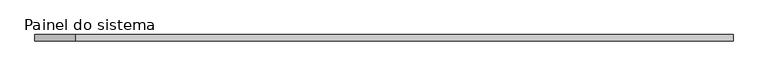
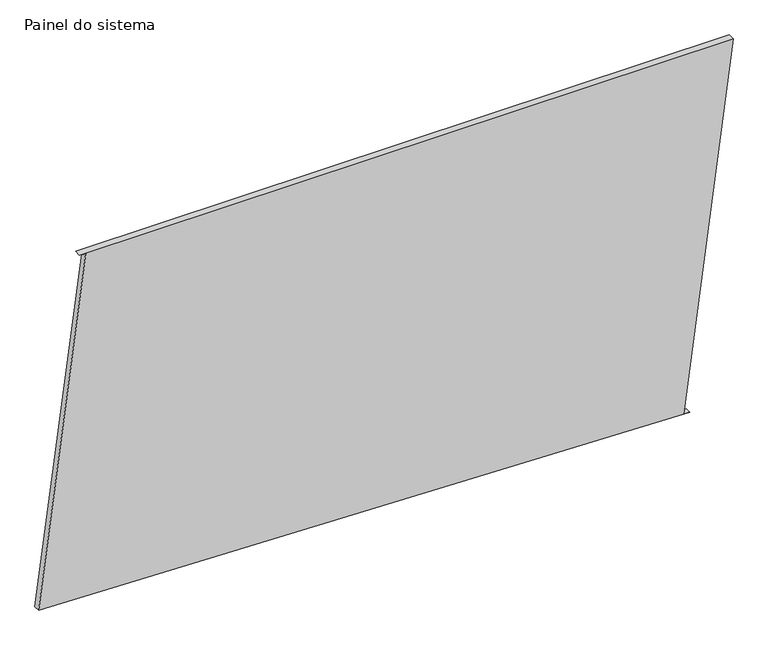
"""IFC4 building model written with IfcOpenShell, lengths in millimetres: plate geometry, Painel do sistema : Envidraçado."""

from ifc_helpers import new_model, si_unit, frame, origin, place, context, project, spatial, polyline, outline, extrude, source, transform, mapped, element, save


def painel_do_sistema_4ceb30a2(model_context):
    return source(origin(), model_context, "Body", "SweptSolid", [
        extrude(outline(polyline([(0.0, 1194.9263795), (3.2380023, 1170.1369595), (1493.6080059, 1364.8095843), (1493.6080059, -1204.4608379), (1490.3700036, -1179.6714179), (72.9936776, -1364.8095843), (0.0, 1194.9263795)])), frame((0.0, 24.5, 0.0), z_axis=(0.0, 1.0, 0.0), x_axis=(0.0, 0.0, 1.0)), (0.0, 0.0, 1.0), 25.0),
    ])


if __name__ == "__main__":
    model = new_model("IFC4")
    model_context = context("Model", 3, world=origin())
    ifc_project = project(units=[si_unit("LENGTHUNIT", "METRE", prefix="MILLI")], contexts=[model_context])
    site = spatial("IfcSite", under=ifc_project)
    building = spatial("IfcBuilding", under=site)
    placement = place(None, origin())
    painel_do_sistema_shape = painel_do_sistema_4ceb30a2(model_context)
    element("IfcPlate", 1, ObjectType="Painel do sistema : Envidraçado", at=placement, inside=building, context=model_context, shape_type="MappedRepresentation", body=[
        mapped(painel_do_sistema_shape, transform((0.0, 0.0, 0.0), x_axis=(1.0, 0.0, 0.0), y_axis=(0.0, 1.0, 0.0), z_axis=(0.0, 0.0, 1.0))),
    ])
    save(model, "model.ifc")

# Revit data of these elements
# Type "Painel do sistema : Envidraçado"
#   Construction Type Id = "GSP4R"
#   Analytic Construction = "Vidraça única Pilkington 1/8 pol"
#   Visual Light Transmittance = 0.9
#   Solar Heat Gain Coefficient = 0.86
#   Heat Transfer Coefficient (U) = 6.7069 W/(m²·K)
# Element 1 (IfcPlate, "Painel do sistema : Envidraçado")
#   Materials on its faces: "Vidro"
# Materials
#   "Vidro": class "Vidro", colour RGB 0 128 192, transparency 0.9, Description = "Vidro de sílica", Cost = 0
